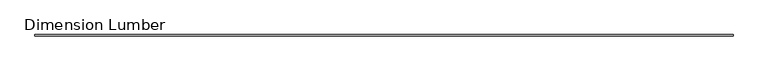
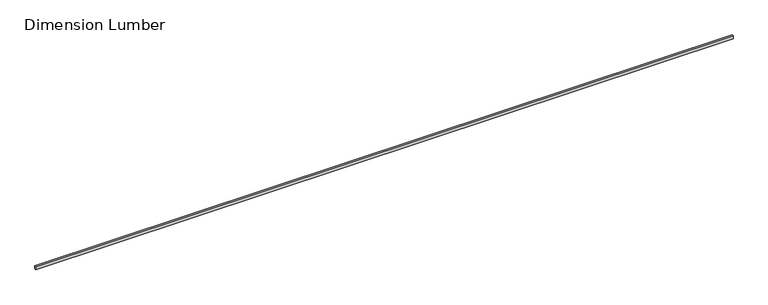
"""IFC4 building model written with IfcOpenShell, lengths in millimetres: beam geometry, Dimension Lumber : Roof Lumbers."""

from ifc_helpers import new_model, si_unit, frame, origin, place, context, project, spatial, polyline, outline, extrude, source, transform, mapped, element, save


def dimension_lumber_bf031064(model_context):
    return source(origin(), model_context, "Body", "SweptSolid", [
        extrude(outline(polyline([(13801.725, 19.05), (13801.725, -19.05), (-5743.575, -19.05), (-5743.575, 19.05), (13801.725, 19.05)])), frame((0.0, 0.0, -44.45), z_axis=(0.0, 0.0, 1.0), x_axis=(1.0, 0.0, 0.0)), (0.0, 0.0, 1.0), 88.9),
    ])


if __name__ == "__main__":
    model = new_model("IFC4")
    model_context = context("Model", 3, world=origin())
    ifc_project = project(units=[si_unit("LENGTHUNIT", "METRE", prefix="MILLI")], contexts=[model_context])
    site = spatial("IfcSite", under=ifc_project)
    building = spatial("IfcBuilding", under=site)
    placement = place(None, origin())
    dimension_lumber_shape = dimension_lumber_bf031064(model_context)
    element("IfcBeam", 1, ObjectType="Dimension Lumber : Roof Lumbers", at=placement, inside=building, context=model_context, shape_type="MappedRepresentation", body=[
        mapped(dimension_lumber_shape, transform((0.0, 0.0, 0.0), x_axis=(1.0, 0.0, 0.0), y_axis=(0.0, 1.0, 0.0), z_axis=(0.0, 0.0, 1.0))),
    ])
    save(model, "model.ifc")

# Revit data of these elements
# Type "Dimension Lumber : Roof Lumbers"
#   Assembly Code = "B10"
#   A = 0.0364583 SF
#   Length [instance default] = 5' - 0"
#   b = 0' - 1 1/2"
#   d = 0' - 3 1/2"
#   Structural Material [instance default] = Softwood, Lumber
# Element 1 (IfcBeam, "Dimension Lumber : Roof Lumbers")
#   Structural Material = Douglas Fir #2
#   Materials on its faces: "Douglas Fir #2"
# Materials
#   "Softwood, Lumber": class "Wood", colour RGB 223 192 134, transparency 0, Description = "Pinus Echinata", Cost = 0
#   "Douglas Fir #2": class "Wood", colour RGB 223 192 134, transparency 0, Description = "Pinus Echinata", Cost = 0
